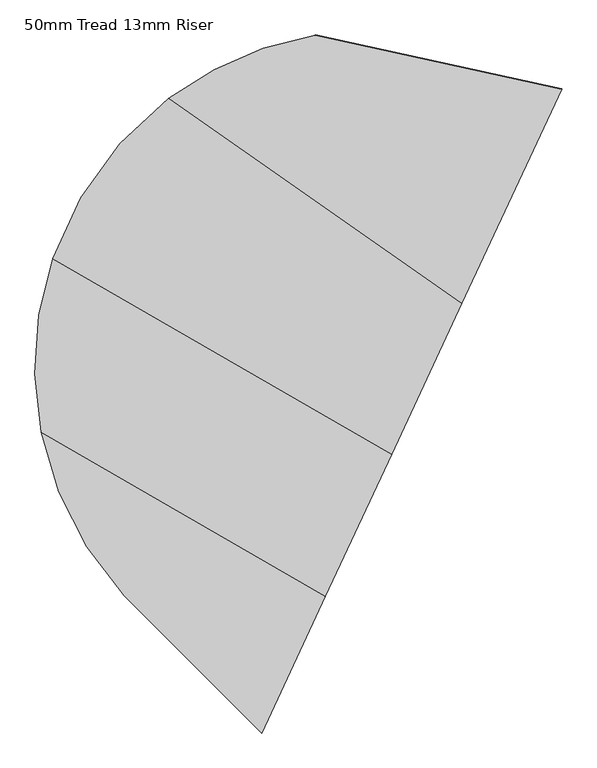
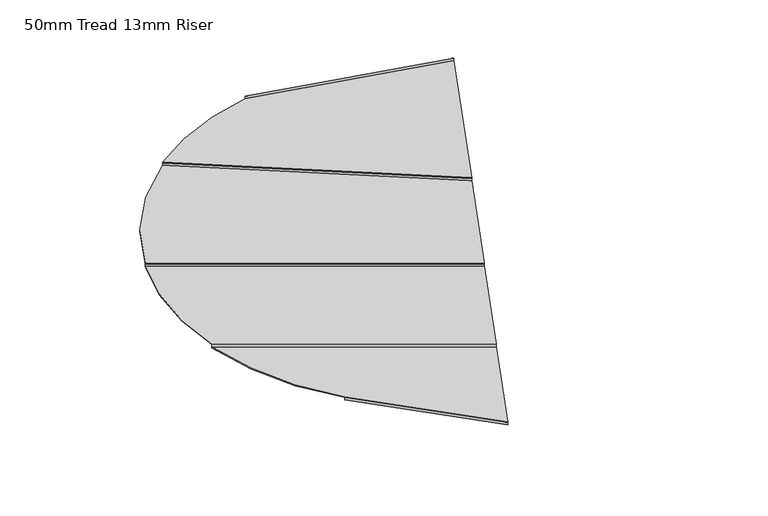
"""IFC4 building model written with IfcOpenShell, lengths in millimetres: stair flight geometry, 50mm Tread 13mm Riser."""

from ifc_helpers import new_model, si_unit, point, frame, frame_2d, origin, place, context, project, spatial, polyline, circle_curve, trimmed, segment, composite_curve, outline, extrude, source, transform, mapped, element, save


def stair_flight_50mm_tread_13mm_riser_9b67f3fa(model_context):
    return source(origin(), model_context, "Body", "SweptSolid", [
        extrude(outline(polyline([(-33951.0721115, -10807.6077739), (-33956.6938735, -10819.6636815), (-39674.1820519, -5102.1755031), (-39665.3432171, -5093.3366684), (-33951.0721115, -10807.6077739)])), frame((0.0, 0.0, 4000.0), z_axis=(0.0, 0.0, 1.0), x_axis=(1.0, 0.0, 0.0)), (0.0, 0.0, 1.0), 136.0465116),
        extrude(outline(composite_curve([segment(polyline([(-43126.7016614, 1700.4461468), (-31301.9611451, -5126.5709734), (-33956.6938735, -10819.6636815), (-39674.1820519, -5102.1755031)]), True, "CONTINUOUS"), segment(trimmed(circle_curve(frame_2d((-29370.8031879, 4404.5113866)), 14019.1551683), [point((-39674.1820519, -5102.1755031))], [point((-43126.7016614, 1700.4461468))], False, "CARTESIAN"), True, "CONTINUOUS")], self_intersect=False)), frame((0.0, 0.0, 4136.0465116), z_axis=(0.0, 0.0, 1.0), x_axis=(1.0, 0.0, 0.0)), (0.0, 0.0, 1.0), 50.0),
        extrude(outline(composite_curve([segment(polyline([(-31296.6582377, -5115.1988517), (-31301.9611451, -5126.5709734), (-43126.7016614, 1700.4461468)]), True, "CONTINUOUS"), segment(trimmed(circle_curve(frame_2d((-29370.8031879, 4404.5113866)), 14019.1551683), [point((-43126.7016614, 1700.4461468))], [point((-43129.8909384, 1716.7212335))], False, "CARTESIAN"), True, "CONTINUOUS"), segment(polyline([(-43129.8909384, 1716.7212335), (-31296.6582377, -5115.1988517)]), True, "CONTINUOUS")], self_intersect=False)), frame((0.0, 0.0, 4136.0465116), z_axis=(0.0, 0.0, 1.0), x_axis=(1.0, 0.0, 0.0)), (0.0, 0.0, 1.0), 186.0465116),
        extrude(outline(composite_curve([segment(polyline([(-42639.6981065, 8929.2367121), (-28542.8295393, 790.40585), (-31301.9611451, -5126.5709734), (-43126.7016614, 1700.4461468)]), True, "CONTINUOUS"), segment(trimmed(circle_curve(frame_2d((-29370.8031879, 4404.5113866)), 14019.1551683), [point((-43126.7016614, 1700.4461468))], [point((-42639.6981065, 8929.2367121))], False, "CARTESIAN"), True, "CONTINUOUS")], self_intersect=False)), frame((0.0, 0.0, 4322.0930233), z_axis=(0.0, 0.0, 1.0), x_axis=(1.0, 0.0, 0.0)), (0.0, 0.0, 1.0), 50.0),
        extrude(outline(composite_curve([segment(polyline([(-28537.5266318, 801.7779717), (-28542.8295393, 790.40585), (-42639.6981065, 8929.2367121)]), True, "CONTINUOUS"), segment(trimmed(circle_curve(frame_2d((-29370.8031879, 4404.5113866)), 14019.1551683), [point((-42639.6981065, 8929.2367121))], [point((-42635.5806752, 8941.2932687))], False, "CARTESIAN"), True, "CONTINUOUS"), segment(polyline([(-42635.5806752, 8941.2932687), (-28537.5266318, 801.7779717)]), True, "CONTINUOUS")], self_intersect=False)), frame((0.0, 0.0, 4322.0930233), z_axis=(0.0, 0.0, 1.0), x_axis=(1.0, 0.0, 0.0)), (0.0, 0.0, 1.0), 186.0465116),
        extrude(outline(composite_curve([segment(polyline([(-37811.70321, 15597.7199726), (-25619.0988702, 7060.3665035), (-28542.8295393, 790.40585), (-42639.6981065, 8929.2367121)]), True, "CONTINUOUS"), segment(trimmed(circle_curve(frame_2d((-29370.8031879, 4404.5113866)), 14019.1551683), [point((-42639.6981065, 8929.2367121))], [point((-37811.70321, 15597.7199726))], False, "CARTESIAN"), True, "CONTINUOUS")], self_intersect=False)), frame((0.0, 0.0, 4508.1395349), z_axis=(0.0, 0.0, 1.0), x_axis=(1.0, 0.0, 0.0)), (0.0, 0.0, 1.0), 50.0),
        extrude(outline(composite_curve([segment(polyline([(-25613.7346474, 7071.8701165), (-25619.0988702, 7060.3665035), (-37811.70321, 15597.7199726)]), True, "CONTINUOUS"), segment(trimmed(circle_curve(frame_2d((-29370.8031879, 4404.5113866)), 14019.1551683), [point((-37811.70321, 15597.7199726))], [point((-37801.2052211, 15605.628884))], False, "CARTESIAN"), True, "CONTINUOUS"), segment(polyline([(-37801.2052211, 15605.628884), (-25613.7346474, 7071.8701165)]), True, "CONTINUOUS")], self_intersect=False)), frame((0.0, 0.0, 4508.1395349), z_axis=(0.0, 0.0, 1.0), x_axis=(1.0, 0.0, 0.0)), (0.0, 0.0, 1.0), 186.0465116),
        extrude(outline(polyline([(-21454.9887913, 15990.3293855), (-21460.4028717, 15978.7188527), (-31719.3733193, 18225.5435467), (-31716.69907, 18237.7541319), (-21454.9887913, 15990.3293855)])), frame((0.0, 0.0, 4694.1860465), z_axis=(0.0, 0.0, 1.0), x_axis=(1.0, 0.0, 0.0)), (0.0, 0.0, 1.0), 186.0465116),
        extrude(outline(composite_curve([segment(polyline([(-31719.3733193, 18225.5435467), (-21460.4028717, 15978.7188527), (-25619.0988702, 7060.3665035), (-37811.70321, 15597.7199726)]), True, "CONTINUOUS"), segment(trimmed(circle_curve(frame_2d((-29370.8031879, 4404.5113866)), 14019.1551683), [point((-37811.70321, 15597.7199726))], [point((-31719.3733193, 18225.5435467))], False, "CARTESIAN"), True, "CONTINUOUS")], self_intersect=False)), frame((0.0, 0.0, 4694.1860465), z_axis=(0.0, 0.0, 1.0), x_axis=(1.0, 0.0, 0.0)), (0.0, 0.0, 1.0), 50.0),
    ])


if __name__ == "__main__":
    model = new_model("IFC4")
    model_context = context("Model", 3, world=origin())
    ifc_project = project(units=[si_unit("LENGTHUNIT", "METRE", prefix="MILLI")], contexts=[model_context])
    site = spatial("IfcSite", under=ifc_project)
    building = spatial("IfcBuilding", under=site)
    placement = place(None, origin())
    stair_flight_50mm_tread_13mm_riser_shape = stair_flight_50mm_tread_13mm_riser_9b67f3fa(model_context)
    element("IfcStairFlight", 1, ObjectType="50mm Tread 13mm Riser", at=placement, inside=building, context=model_context, shape_type="MappedRepresentation", body=[
        mapped(stair_flight_50mm_tread_13mm_riser_shape, transform((0.0, 0.0, 0.0), x_axis=(1.0, 0.0, 0.0), y_axis=(0.0, 1.0, 0.0), z_axis=(0.0, 0.0, 1.0))),
    ])
    save(model, "model.ifc")
